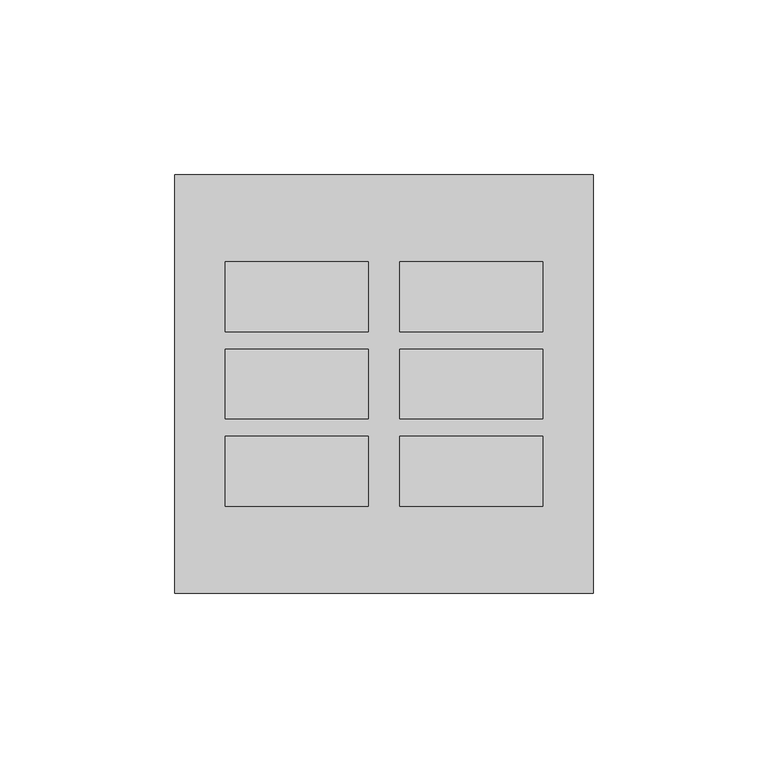
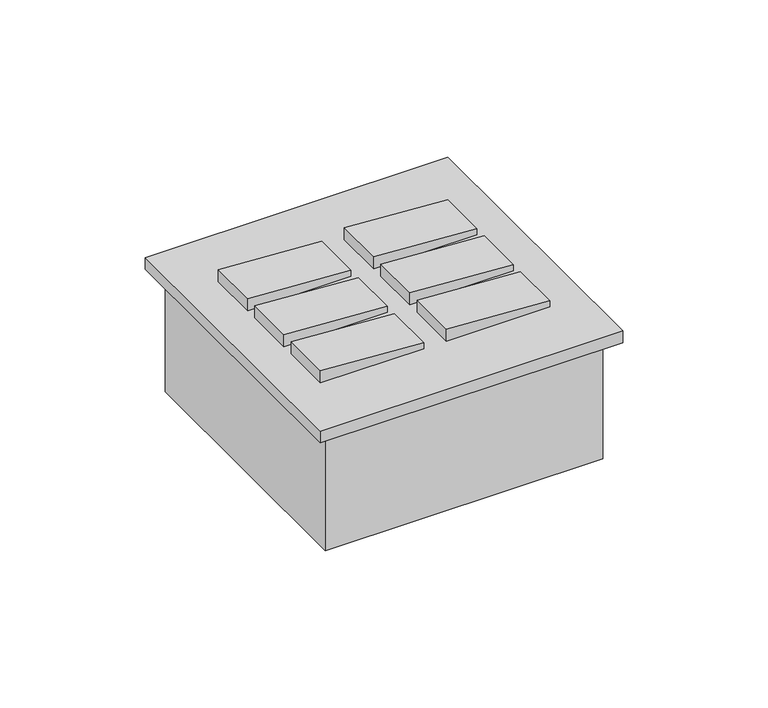
"""IFC4 building model written with IfcOpenShell, lengths in millimetres: proxy geometry, CAIXA VERTICE V7 : Interruptor 6s."""

from ifc_helpers import new_model, si_unit, frame, origin, origin_with_axes, place, context, project, spatial, polyline, outline, extrude, faceted_brep, source, transform, mapped, element, save


def electrical_fixtures_334ea5fa(model_context):
    return source(origin(), model_context, "Body", "SolidModel", [
        extrude(outline(polyline([(5.0, 45.5), (7.5, 45.5), (10.0, 4.5), (5.0, 4.5), (5.0, 45.5)])), frame((0.0, 1065.0, 0.0), z_axis=(0.0, 1.0, 0.0), x_axis=(0.0, 0.0, 1.0)), (0.0, 0.0, 1.0), 20.0),
        extrude(outline(polyline([(5.0, 45.5), (7.5, 45.5), (10.0, 4.5), (5.0, 4.5), (5.0, 45.5)])), frame((0.0, 1090.0, 0.0), z_axis=(0.0, 1.0, 0.0), x_axis=(0.0, 0.0, 1.0)), (0.0, 0.0, 1.0), 20.0),
        extrude(outline(polyline([(5.0, 45.5), (7.5, 45.5), (10.0, 4.5), (5.0, 4.5), (5.0, 45.5)])), frame((0.0, 1115.0, 0.0), z_axis=(0.0, 1.0, 0.0), x_axis=(0.0, 0.0, 1.0)), (0.0, 0.0, 1.0), 20.0),
        extrude(outline(polyline([(5.0, -4.5), (7.5, -4.5), (10.0, -45.5), (5.0, -45.5), (5.0, -4.5)])), frame((0.0, 1065.0, 0.0), z_axis=(0.0, 1.0, 0.0), x_axis=(0.0, 0.0, 1.0)), (0.0, 0.0, 1.0), 20.0),
        extrude(outline(polyline([(5.0, -4.5), (7.5, -4.5), (10.0, -45.5), (5.0, -45.5), (5.0, -4.5)])), frame((0.0, 1090.0, 0.0), z_axis=(0.0, 1.0, 0.0), x_axis=(0.0, 0.0, 1.0)), (0.0, 0.0, 1.0), 20.0),
        extrude(outline(polyline([(5.0, -4.5), (7.5, -4.5), (10.0, -45.5), (5.0, -45.5), (5.0, -4.5)])), frame((0.0, 1115.0, 0.0), z_axis=(0.0, 1.0, 0.0), x_axis=(0.0, 0.0, 1.0)), (0.0, 0.0, 1.0), 20.0),
        faceted_brep([(55.0, 1155.0, 0.0), (-55.0, 1155.0, 0.0), (-55.0, 1045.0, 0.0), (55.0, 1045.0, 0.0), (53.0, 1153.0, 0.0), (53.0, 1047.0, 0.0), (-53.0, 1047.0, 0.0), (-53.0, 1153.0, 0.0), (53.0, 1047.0, -48.0), (53.0, 1153.0, -48.0), (-53.0, 1153.0, -48.0), (-53.0, 1047.0, -48.0), (55.0, 1155.0, -50.0), (55.0, 1045.0, -50.0), (-55.0, 1045.0, -50.0), (-55.0, 1155.0, -50.0)], [[[0, 1, 2, 3], [4, 5, 6, 7]], [[8, 9, 10, 11]], [[12, 13, 14, 15]], [[12, 15, 1, 0]], [[1, 15, 14, 2]], [[2, 14, 13, 3]], [[3, 13, 12, 0]], [[5, 4, 9, 8]], [[6, 5, 8, 11]], [[7, 6, 11, 10]], [[4, 7, 10, 9]]]),
        extrude(outline(polyline([(60.0, 1160.0), (60.0, 1040.0), (-60.0, 1040.0), (-60.0, 1160.0), (60.0, 1160.0)])), origin_with_axes(), (0.0, 0.0, 1.0), 5.0),
    ])


if __name__ == "__main__":
    model = new_model("IFC4")
    model_context = context("Model", 3, world=origin())
    ifc_project = project(units=[si_unit("LENGTHUNIT", "METRE", prefix="MILLI")], contexts=[model_context])
    site = spatial("IfcSite", under=ifc_project)
    building = spatial("IfcBuilding", under=site)
    placement = place(None, origin())
    electrical_fixtures_shape = electrical_fixtures_334ea5fa(model_context)
    element("IfcBuildingElementProxy", 1, Name="CAIXA VERTICE V7 : Interruptor 6s", ObjectType="CAIXA VERTICE V7 : Interruptor 6s", at=placement, inside=building, context=model_context, shape_type="MappedRepresentation", body=[
        mapped(electrical_fixtures_shape, transform((0.0, 0.0, 0.0), x_axis=(1.0, 0.0, 0.0), y_axis=(0.0, 1.0, 0.0), z_axis=(0.0, 0.0, 1.0))),
    ])
    save(model, "model.ifc")

# Revit data of these elements
# Type "CAIXA VERTICE V7 : Interruptor 6s"
#   URL = "www.facebook.com/verticetreinamentos"
#   SEÇÃO [instance default] = ""
#   Rotação [instance default] = 0.00°
#   LARGURA DA TAMPA = 0.08 m
#   BORDA = 0.01 m
#   ALTURA DE INSTALAÇÃO [instance default] = 1.10 m
#   Distância Anotação [instance default] = 0.0015 m
#   ALTURA DA TAMPA = 0.12 m
#   Vertical [instance default] = yes
#   VER SEÇÃO [instance default] = yes
#   SHADE ESQ [instance default] = no
#   SHADE DIR [instance default] = yes
#   HORIZONTAL [instance default] = no
#   ANDAR COM A LEGENDA [instance default] = 0
#   Material Tampa [instance default] = Plástico, branco opaco
#   Caixa = element 1798508
#   Anotação = element 1798523
#   Default Elevation = 0
# Element 1 (IfcBuildingElementProxy, "CAIXA VERTICE V7 : Interruptor 6s")
#   SEÇÃO = "6"
#   Materials on its faces: "Plástico, branco opaco"
# Materials
#   "Plástico, branco opaco": class "Plástico", colour RGB 120 120 120, transparency 0, Description = "Plastic, generic, opaque white", Cost = 0
